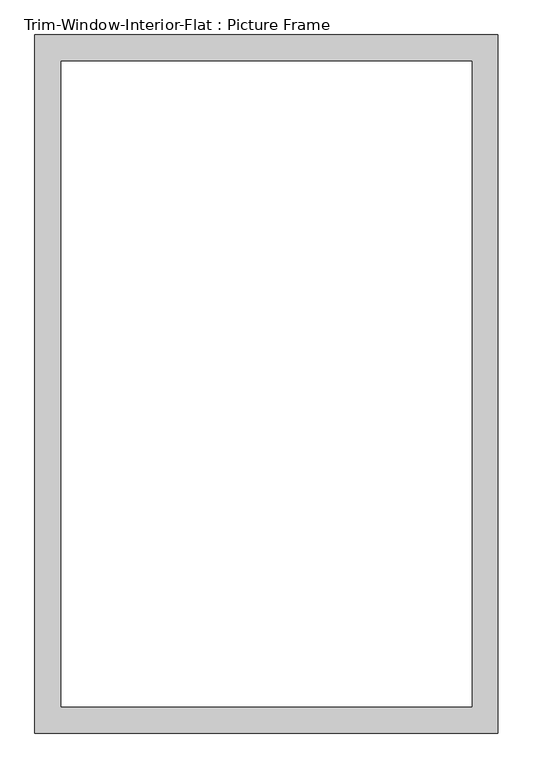
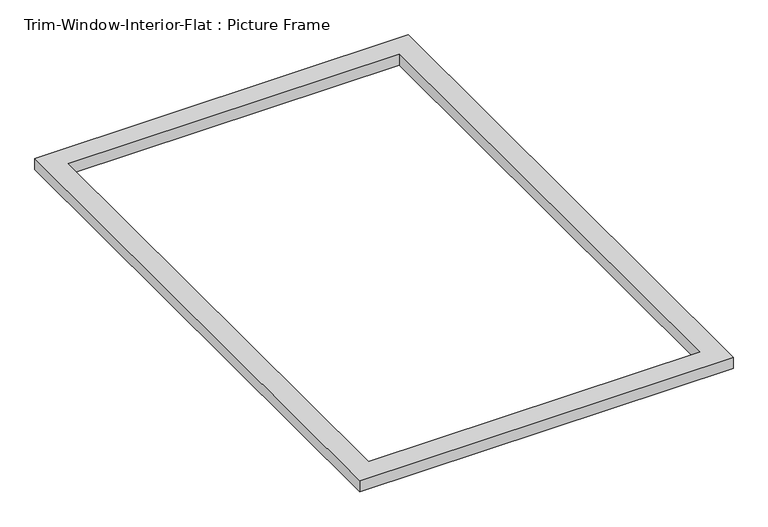
"""IFC4 building model written with IfcOpenShell, lengths in millimetres: proxy geometry, Trim-Window-Interior-Flat : Picture Frame."""

from ifc_helpers import new_model, si_unit, origin, origin_with_axes, place, context, project, spatial, polyline, outline, extrude, source, transform, mapped, element, save


def trim_window_interior_flat_picture_frame_b9635a36(model_context):
    return source(origin(), model_context, "Body", "SweptSolid", [
        extrude(outline(polyline([(501.65, -44.45), (-501.65, -44.45), (-501.65, 1466.85), (501.65, 1466.85), (501.65, -44.45)]), holes=[polyline([(444.5, 12.7), (444.5, 1409.7), (-444.5, 1409.7), (-444.5, 12.7), (444.5, 12.7)])]), origin_with_axes(), (0.0, 0.0, 1.0), 31.75),
    ])


if __name__ == "__main__":
    model = new_model("IFC4")
    model_context = context("Model", 3, world=origin())
    ifc_project = project(units=[si_unit("LENGTHUNIT", "METRE", prefix="MILLI")], contexts=[model_context])
    site = spatial("IfcSite", under=ifc_project)
    building = spatial("IfcBuilding", under=site)
    placement = place(None, origin())
    trim_window_interior_flat_picture_frame_shape = trim_window_interior_flat_picture_frame_b9635a36(model_context)
    element("IfcBuildingElementProxy", 1, Name="Trim-Window-Interior-Flat : Picture Frame", ObjectType="Trim-Window-Interior-Flat : Picture Frame", at=placement, inside=building, context=model_context, shape_type="MappedRepresentation", body=[
        mapped(trim_window_interior_flat_picture_frame_shape, transform((0.0, 0.0, 0.0), x_axis=(1.0, 0.0, 0.0), y_axis=(0.0, 1.0, 0.0), z_axis=(0.0, 0.0, 1.0))),
    ])
    save(model, "model.ifc")

# Revit data of these elements
# Type "Trim-Window-Interior-Flat : Picture Frame"
#   Trim Thickness_Picture Frame = 0' - 1 1/4"
#   Trim Width = 0' - 2 1/4"
#   Trim Thickness_with Sill = 0' - 0 3/4"
#   Sill Thickness = 0' - 1 1/4"
#   Opening Width [instance default] = 2' - 0"
#   Opening Height [instance default] = 3' - 0"
#   Default Elevation = 4' - 0"
#   Sill = no
#   Picture Frame = yes
#   Trim Material [instance default] = none
# Element 1 (IfcBuildingElementProxy, "Trim-Window-Interior-Flat : Picture Frame")
#   Opening Width = 3' - 0"
#   Opening Height = 4' - 8"
#   Trim Material = Wood - Stained
#   Materials on its faces: "Wood - Stained"
# Materials
#   "Wood - Stained": class "Wood", colour RGB 224 178 126, transparency 0, Cost = 0
